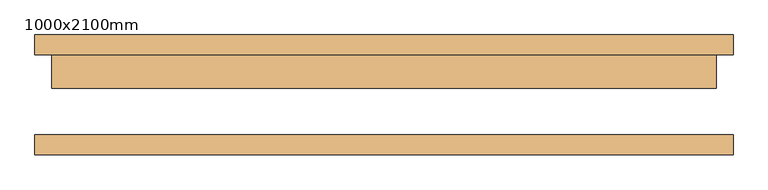
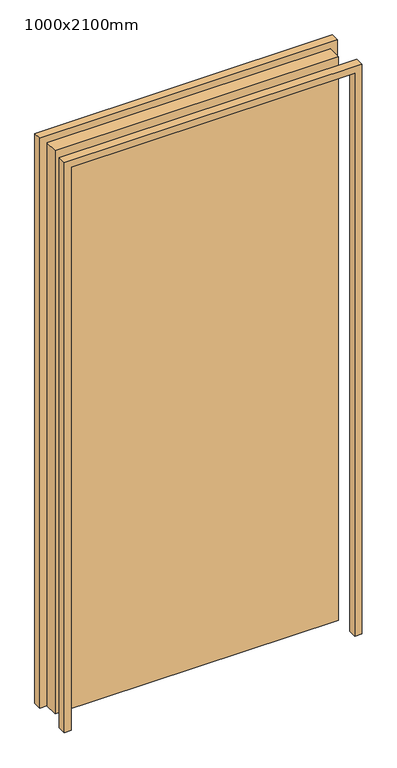
"""IFC4 building model written with IfcOpenShell, lengths in millimetres: door geometry, WWm-SingleSolid-Flush : 1000x2100mm."""

from ifc_helpers import new_model, si_unit, frame, origin, origin_with_axes, place, context, project, spatial, polyline, outline, extrude, source, transform, mapped, element, save


def door_1000x2100mm_6e1781e5(model_context):
    return source(origin(), model_context, "Body", "SweptSolid", [
        extrude(outline(polyline([(2125.0, -525.0), (0.0, -525.0), (0.0, -500.0), (2100.0, -500.0), (2100.0, 500.0), (0.0, 500.0), (0.0, 525.0), (2125.0, 525.0), (2125.0, -525.0)])), frame((0.0, 60.0, 0.0), z_axis=(0.0, 1.0, 0.0), x_axis=(0.0, 0.0, 1.0)), (0.0, 0.0, 1.0), 30.0),
        extrude(outline(polyline([(2125.0, 525.0), (2125.0, -525.0), (0.0, -525.0), (0.0, -500.0), (2100.0, -500.0), (2100.0, 500.0), (0.0, 500.0), (0.0, 525.0), (2125.0, 525.0)])), frame((0.0, -90.0, 0.0), z_axis=(0.0, 1.0, 0.0), x_axis=(0.0, 0.0, 1.0)), (0.0, 0.0, 1.0), 30.0),
        extrude(outline(polyline([(500.0, 10.0), (-500.0, 10.0), (-500.0, 60.0), (500.0, 60.0), (500.0, 10.0)])), origin_with_axes(), (0.0, 0.0, 1.0), 2100.0),
    ])


if __name__ == "__main__":
    model = new_model("IFC4")
    model_context = context("Model", 3, world=origin())
    ifc_project = project(units=[si_unit("LENGTHUNIT", "METRE", prefix="MILLI")], contexts=[model_context])
    site = spatial("IfcSite", under=ifc_project)
    building = spatial("IfcBuilding", under=site)
    placement = place(None, origin())
    door_1000x2100mm_shape = door_1000x2100mm_6e1781e5(model_context)
    element("IfcDoor", 1, ObjectType="WWm-SingleSolid-Flush : 1000x2100mm", at=placement, inside=building, context=model_context, shape_type="MappedRepresentation", body=[
        mapped(door_1000x2100mm_shape, transform((0.0, 0.0, 0.0), x_axis=(1.0, 0.0, 0.0), y_axis=(0.0, 1.0, 0.0), z_axis=(0.0, 0.0, 1.0))),
    ])
    save(model, "model.ifc")

# Revit data of these elements
# Type "WWm-SingleSolid-Flush : 1000x2100mm"
#   Type Mark = "EX1-51"
#   Construction Type Id = "MDOOR"
#   Assembly Code = "C1020"
#   Analytic Construction = "Metal"
#   Thickness = 50 mm
#   Thermal Resistance (R) = 0.270117 (m²·K)/W
#   Heat Transfer Coefficient (U) = 3.7021 W/(m²·K)
#   Height = 2100 mm
#   Trim Projection Ext = 30 mm
#   Trim Projection Int = 30 mm
#   Trim Width = 25 mm
#   Width = 1000 mm
#   Not 90 Degree [instance default] = no
#   90 Degree [instance default] = yes
#   Door Material = WW-EC-RGB-White
#   Frame Material = WW-EC-RGB-White
#   Visual Light Transmittance = 0
#   Solar Heat Gain Coefficient = 0
#   Function = (empty or 0)
#   Wall Closure = (empty or 0)
# Element 1 (IfcDoor, "WWm-SingleSolid-Flush : 1000x2100mm")
#   Materials on its faces: "WW-EC-RGB-White"
# Materials
#   "WW-EC-RGB-White": class "Generic", colour RGB 255 255 255, transparency 0, Comments = "If region requests off-white, swith asset color to RGB 231-228-220", Description = "Generic Color", Cost = 0
